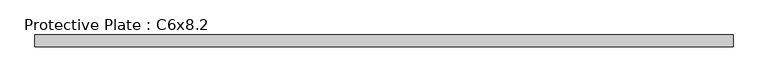
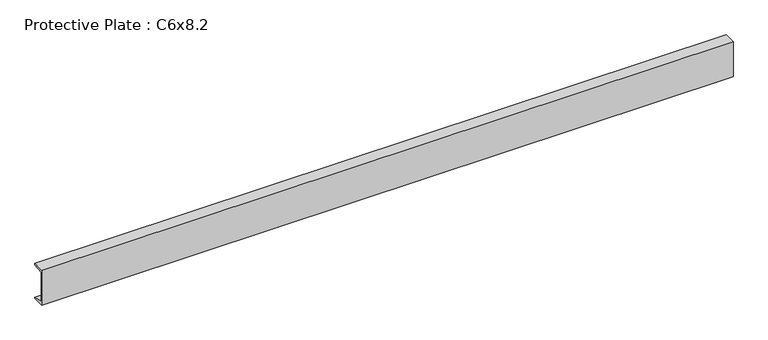
"""IFC4 building model written with IfcOpenShell, lengths in millimetres: proxy geometry, Protective Plate : C6x8.2."""

from ifc_helpers import new_model, si_unit, frame, origin, place, context, project, spatial, polyline, outline, extrude, source, transform, mapped, element, save


def protective_plate_c6x8_2_5f1a67c2(model_context):
    return source(origin(), model_context, "Body", "SweptSolid", [
        extrude(outline(polyline([(-531775.7413841, 914.4), (-531775.7413841, 909.32), (-531819.4492278, 901.6131279), (-531819.4492278, 774.7868721), (-531775.7413841, 767.08), (-531775.7413841, 762.0), (-531824.5093841, 762.0), (-531824.5093841, 914.4), (-531775.7413841, 914.4)])), frame((587416.6934739, 0.0, 0.0), z_axis=(1.0, 0.0, 0.0), x_axis=(0.0, 1.0, 0.0)), (0.0, 0.0, 1.0), 2854.7900527),
    ])


if __name__ == "__main__":
    model = new_model("IFC4")
    model_context = context("Model", 3, world=origin())
    ifc_project = project(units=[si_unit("LENGTHUNIT", "METRE", prefix="MILLI")], contexts=[model_context])
    site = spatial("IfcSite", under=ifc_project)
    building = spatial("IfcBuilding", under=site)
    placement = place(None, origin())
    protective_plate_c6x8_2_shape = protective_plate_c6x8_2_5f1a67c2(model_context)
    element("IfcBuildingElementProxy", 1, Name="Protective Plate : C6x8.2", ObjectType="Protective Plate : C6x8.2", at=placement, inside=building, context=model_context, shape_type="MappedRepresentation", body=[
        mapped(protective_plate_c6x8_2_shape, transform((0.0, 0.0, 0.0), x_axis=(1.0, 0.0, 0.0), y_axis=(0.0, 1.0, 0.0), z_axis=(0.0, 0.0, 1.0))),
    ])
    save(model, "model.ifc")

# Revit data of these elements
# Element 1 (IfcBuildingElementProxy, "Protective Plate : C6x8.2")
#   Materials on its faces: "C6x8.2 GALV CHANNEL"
# Materials
#   "C6x8.2 GALV CHANNEL": class "Generic", colour RGB 211 211 207, transparency 0, Cost = 0
